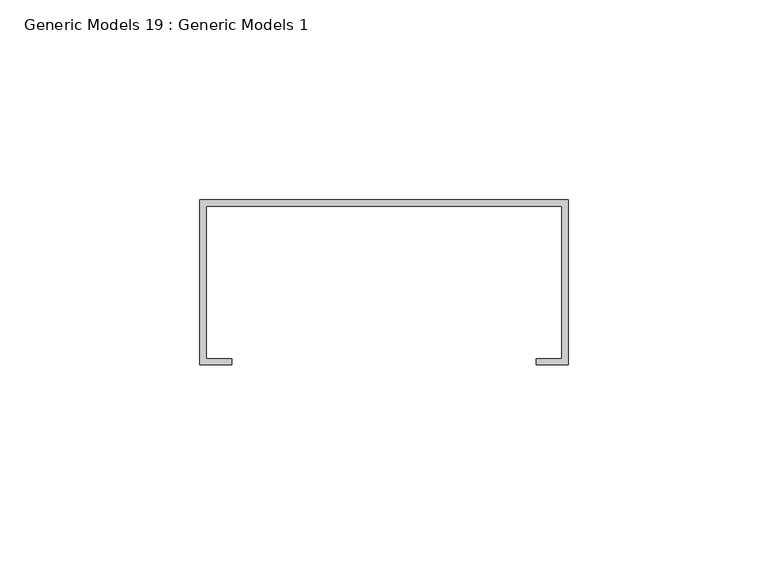
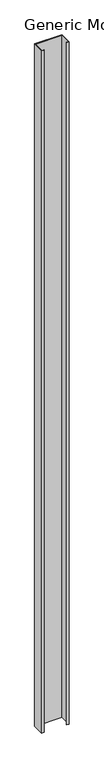
"""IFC4 building model written with IfcOpenShell, lengths in millimetres: proxy geometry, Generic Models 19 : Generic Models 1."""

import ifcopenshell
import ifcopenshell.guid

model = None  # the IFC model being written
_history = None  # IfcOwnerHistory: only IFC2X3 demands one
_inside = {}  # id of a spatial element -> (the spatial element, [elements in it])
_under = {}  # id of a project, library or spatial element -> (it, [spatial elements below it])
_declared = {}  # id of a project -> (the project, [libraries it declares])
_typed = {}  # id of a type object -> (the type object, [elements of that type])
_made_of = {}  # id of a material, layer set ... -> (it, [elements and type objects made of it])


def new_model(schema):
    """Start an empty IFC model of exactly this schema.

    Asked for "IFC4X3", IfcOpenShell would pick the latest addendum, in which some entities
    have other attributes; the version numbers below select the first issue.
    IFC2X3 requires an IfcOwnerHistory on every rooted entity: one is made here for all.
    """
    global model, _history
    if schema == "IFC4X3":
        model = ifcopenshell.file(schema_version=(4, 3, 0, 0))
    else:
        model = ifcopenshell.file(schema=schema)
    _inside.clear()
    _under.clear()
    _declared.clear()
    _typed.clear()
    _made_of.clear()
    _history = None
    if model.schema == "IFC2X3":
        org = make("IfcOrganization", Name="unknown")
        user = make(
            "IfcPersonAndOrganization",
            ThePerson=make("IfcPerson", FamilyName="unknown"),
            TheOrganization=org,
        )
        app = make(
            "IfcApplication",
            ApplicationDeveloper=org,
            Version="unknown",
            ApplicationFullName="unknown",
            ApplicationIdentifier="unknown",
        )
        _history = make(
            "IfcOwnerHistory",
            OwningUser=user,
            OwningApplication=app,
            ChangeAction="ADDED",
            CreationDate=0,
        )
    return model


def make(cls, **values):
    """One entity of the class cls with the attributes given. An attribute that is None is left unset."""
    return model.create_entity(
        cls, **{name: value for name, value in values.items() if value is not None}
    )


def rooted(cls, **values):
    """An entity with a GlobalId (a new one), such as an element, a storey or a relation."""
    return make(cls, GlobalId=ifcopenshell.guid.new(), OwnerHistory=_history, **values)


def si_unit(unit_type, name, prefix=None):
    """IfcSIUnit, for example si_unit("LENGTHUNIT", "METRE", prefix="MILLI")."""
    return make("IfcSIUnit", UnitType=unit_type, Prefix=prefix, Name=name)


def assignment(units):
    """IfcUnitAssignment: the units of a project."""
    return None if units is None else make("IfcUnitAssignment", Units=units)


def point(xyz):
    """IfcCartesianPoint."""
    return None if xyz is None else make("IfcCartesianPoint", Coordinates=xyz)


def direction(xyz):
    """IfcDirection."""
    return None if xyz is None else make("IfcDirection", DirectionRatios=xyz)


def frame(location, z_axis=None, x_axis=None):
    """IfcAxis2Placement3D, a coordinate frame: its origin and axes. An axis left out is left unset."""
    return make(
        "IfcAxis2Placement3D",
        Location=point(location),
        Axis=direction(z_axis),
        RefDirection=direction(x_axis),
    )


def origin():
    """The frame at (0, 0, 0) with its axes left unset."""
    return frame((0.0, 0.0, 0.0))


def place(relative_to, where):
    """IfcLocalPlacement: puts the frame where relative to a parent placement (None: the world)."""
    return make(
        "IfcLocalPlacement", PlacementRelTo=relative_to, RelativePlacement=where
    )


def context(
    kind, dimensions, precision=None, world=None, true_north=None, identifier=None
):
    """IfcGeometricRepresentationContext, for example the 3D "Model" context."""
    return make(
        "IfcGeometricRepresentationContext",
        ContextIdentifier=identifier,
        ContextType=kind,
        CoordinateSpaceDimension=dimensions,
        Precision=precision,
        WorldCoordinateSystem=world,
        TrueNorth=true_north,
    )


def project(units=None, contexts=None):
    """IfcProject with its units and contexts."""
    return rooted(
        "IfcProject",
        Name="project",
        RepresentationContexts=contexts,
        UnitsInContext=assignment(units),
    )


def spatial(cls, under=None, at=None, **own):
    """A site, building, storey or space (cls), placed at a placement, below another one or the project."""
    s = rooted(cls, ObjectPlacement=at, **own)
    if under is not None:
        _under.setdefault(under.id(), (under, []))[1].append(s)
    return s


def polyline(points):
    """IfcPolyline through the points."""
    return make("IfcPolyline", Points=[point(p) for p in points])


def outline(outer, holes=None, kind="AREA"):
    """IfcArbitraryClosedProfileDef: a profile drawn as a closed curve; with holes, ...WithVoids."""
    if holes is None:
        return make("IfcArbitraryClosedProfileDef", ProfileType=kind, OuterCurve=outer)
    return make(
        "IfcArbitraryProfileDefWithVoids",
        ProfileType=kind,
        OuterCurve=outer,
        InnerCurves=holes,
    )


def extrude(swept, where, along, depth):
    """IfcExtrudedAreaSolid: the profile swept, set in the frame where, extruded along a direction by depth."""
    return make(
        "IfcExtrudedAreaSolid",
        SweptArea=swept,
        Position=where,
        ExtrudedDirection=direction(along),
        Depth=depth,
    )


def shape(context_of_items, identifier, shape_type, items):
    """IfcShapeRepresentation: the items that make up one representation, for example the "Body"."""
    return make(
        "IfcShapeRepresentation",
        ContextOfItems=context_of_items,
        RepresentationIdentifier=identifier,
        RepresentationType=shape_type,
        Items=items,
    )


def source(mapping_origin, context_of_items, identifier, shape_type, items):
    """IfcRepresentationMap: a shape defined once, which mapped items show again and again."""
    return make(
        "IfcRepresentationMap",
        MappingOrigin=mapping_origin,
        MappedRepresentation=shape(context_of_items, identifier, shape_type, items),
    )


def transform(
    local_origin,
    x_axis=None,
    y_axis=None,
    z_axis=None,
    scale=None,
    scale2=None,
    scale3=None,
    uniform=True,
):
    """IfcCartesianTransformationOperator3D, or its non-uniform kind. x_axis, y_axis, z_axis: its Axis1, 2, 3."""
    if uniform:
        return make(
            "IfcCartesianTransformationOperator3D",
            Axis1=direction(x_axis),
            Axis2=direction(y_axis),
            LocalOrigin=point(local_origin),
            Scale=scale,
            Axis3=direction(z_axis),
        )
    return make(
        "IfcCartesianTransformationOperator3DnonUniform",
        Axis1=direction(x_axis),
        Axis2=direction(y_axis),
        LocalOrigin=point(local_origin),
        Scale=scale,
        Axis3=direction(z_axis),
        Scale2=scale2,
        Scale3=scale3,
    )


def mapped(mapping_source, mapping_target):
    """IfcMappedItem: shows the shape of a source again, moved by a transform."""
    return make(
        "IfcMappedItem", MappingSource=mapping_source, MappingTarget=mapping_target
    )


def made_of(thing, what):
    """Note that an element or type object is made of a material, layer set ...; save() writes the relation."""
    if what is not None:
        _made_of.setdefault(what.id(), (what, []))[1].append(thing)
    return thing


def element(
    cls,
    number,
    at=None,
    inside=None,
    cuts=None,
    type_object=None,
    material=None,
    context=None,
    identifier="Body",
    shape_type=None,
    held_by="IfcProductDefinitionShape",
    body=None,
    shapes=None,
    **own,
):
    """One element of the class cls, such as IfcWall. Its Tag is "e" and its number.

    at: its placement. inside: the storey or other place that contains it. cuts: it is an
    opening in that element (IfcRelVoidsElement). A single representation is given by context,
    identifier, shape_type and body (its items); several are given by shapes. held_by: the class
    of the entity that holds the representations. save() writes the other relations.
    """
    e = rooted(cls, Tag="e%d" % number, ObjectPlacement=at, **own)
    if body is not None:
        shapes = [shape(context, identifier, shape_type, body)]
    if shapes is not None:
        e.Representation = make(held_by, Representations=shapes)
    if inside is not None:
        _inside.setdefault(inside.id(), (inside, []))[1].append(e)
    if cuts is not None:
        rooted(
            "IfcRelVoidsElement", RelatingBuildingElement=cuts, RelatedOpeningElement=e
        )
    if type_object is not None:
        _typed.setdefault(type_object.id(), (type_object, []))[1].append(e)
    return made_of(e, material)


def aggregate(whole, parts):
    """IfcRelAggregates: a whole, such as a stair, and the parts it consists of."""
    return rooted("IfcRelAggregates", RelatingObject=whole, RelatedObjects=parts)


def save(model, path):
    """Write the relations noted so far, then the file.

    IfcRelAggregates (storeys below a building ...), IfcRelContainedInSpatialStructure (elements
    in a storey), IfcRelDefinesByType, IfcRelAssociatesMaterial and IfcRelDeclares: one each for
    every whole, place, type object, material and project.
    """
    for whole, parts in _under.values():
        aggregate(whole, parts)
    for where, things in _inside.values():
        rooted(
            "IfcRelContainedInSpatialStructure",
            RelatedElements=things,
            RelatingStructure=where,
        )
    for kind, things in _typed.values():
        rooted("IfcRelDefinesByType", RelatedObjects=things, RelatingType=kind)
    for what, things in _made_of.values():
        rooted("IfcRelAssociatesMaterial", RelatedObjects=things, RelatingMaterial=what)
    for by, libraries in _declared.values():
        rooted("IfcRelDeclares", RelatingContext=by, RelatedDefinitions=libraries)
    model.write(path)


def generic_models_19_generic_models_1_274f06fa(model_context):
    return source(origin(), model_context, "Body", "SweptSolid", [
        extrude(outline(polyline([(49691.925, 630.2375), (49784.0, 630.2375), (49784.0, 588.9625), (49776.0625, 588.9625), (49776.0625, 590.55), (49782.4125, 590.55), (49782.4125, 628.65), (49693.5125, 628.65), (49693.5125, 590.55), (49699.8625, 590.55), (49699.8625, 588.9625), (49691.925, 588.9625), (49691.925, 630.2375)])), frame((0.0, 0.0, 1.5875), z_axis=(0.0, 0.0, 1.0), x_axis=(1.0, 0.0, 0.0)), (0.0, 0.0, 1.0), 2428.875),
    ])


if __name__ == "__main__":
    model = new_model("IFC4")
    model_context = context("Model", 3, world=origin())
    ifc_project = project(units=[si_unit("LENGTHUNIT", "METRE", prefix="MILLI")], contexts=[model_context])
    site = spatial("IfcSite", under=ifc_project)
    building = spatial("IfcBuilding", under=site)
    placement = place(None, origin())
    generic_models_19_generic_models_1_shape = generic_models_19_generic_models_1_274f06fa(model_context)
    element("IfcBuildingElementProxy", 1, Name="Generic Models 19 : Generic Models 1", ObjectType="Generic Models 19 : Generic Models 1", at=placement, inside=building, context=model_context, shape_type="MappedRepresentation", body=[
        mapped(generic_models_19_generic_models_1_shape, transform((0.0, 0.0, 0.0), x_axis=(1.0, 0.0, 0.0), y_axis=(0.0, 1.0, 0.0), z_axis=(0.0, 0.0, 1.0))),
    ])
    save(model, "model.ifc")

# Revit data of these elements
# Element 1 (IfcBuildingElementProxy, "Generic Models 19 : Generic Models 1")
#   Materials on its faces: "METAL STUDS (MATCH EXISTING SIZE/GAUGE/SPACING)"
# Materials
#   "METAL STUDS (MATCH EXISTING SIZE/GAUGE/SPACING)": class "Unassigned", colour RGB 210 209 208, transparency 0, Keynote = "M05121300.02", Cost = 0
